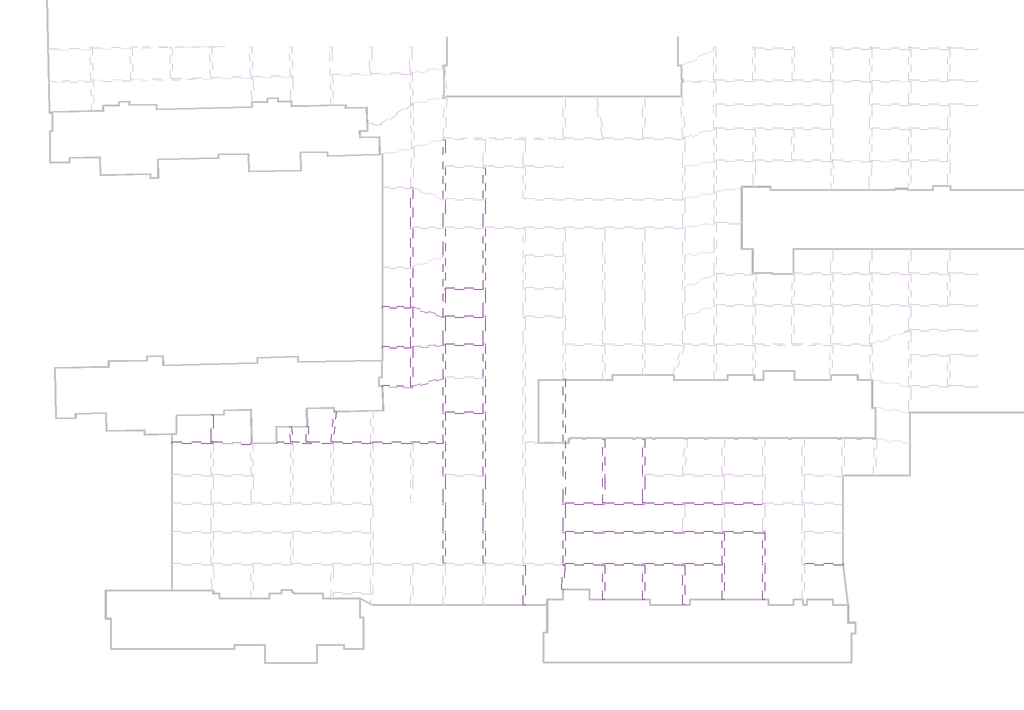
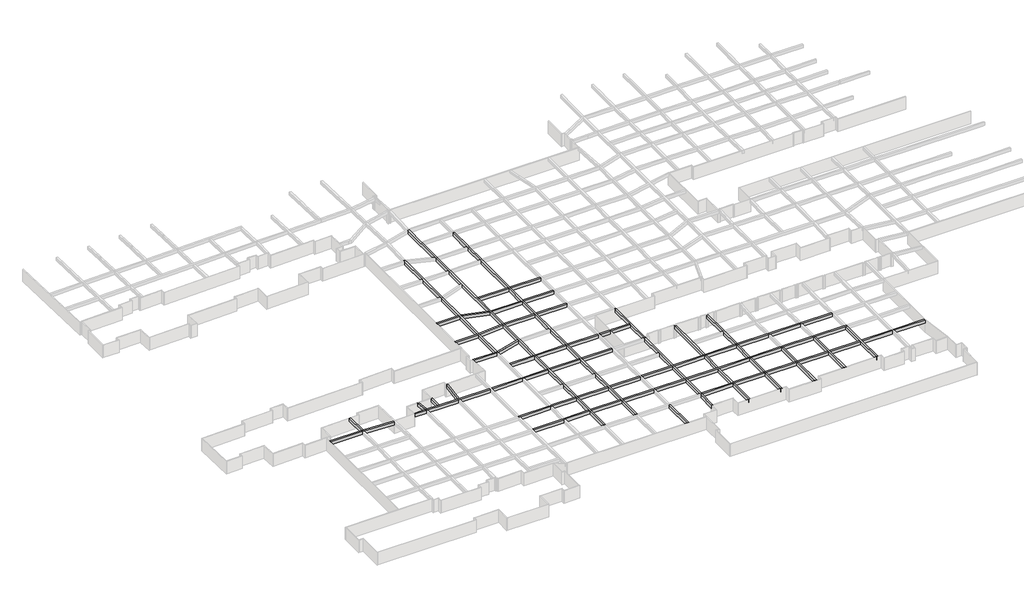
# One storey, part 9 of 20: 35 beams.
"""IFC4 building model written with IfcOpenShell, lengths in millimetres."""

from ifc_helpers import new_model, si_unit, frame, origin, place, context, project, spatial, polyline, outline, extrude, faceted_brep, element, save

model = new_model("IFC4")

# Units and contexts
model_context = context("Model", 3, world=origin())
ifc_project = project(units=[si_unit("LENGTHUNIT", "METRE", prefix="MILLI")], contexts=[model_context])

# Site, building, storey
site = spatial("IfcSite", under=ifc_project)
building = spatial("IfcBuilding", under=site)
storey = spatial("IfcBuildingStorey", under=building, Name="户型图", Elevation=0.0)

# Beams
placement = place(None, origin())
element("IfcBeam", 1, ObjectType="混凝土 - 矩形梁 : KL_beam", at=placement, inside=storey, context=model_context, shape_type="Brep", body=[
    faceted_brep([(62850.0, 87660.0, 3300.0), (62450.0, 87660.0, 3300.0), (62450.0, 81510.0, 3300.0), (62450.0, 81110.0, 3300.0), (62450.0, 75860.0, 3300.0), (62450.0, 75460.0, 3300.0), (62450.0, 63660.0, 3300.0), (62450.0, 63260.0, 3300.0), (62450.0, 57960.0, 3300.0), (62450.0, 57560.0, 3300.0), (62450.0, 52365.0, 3300.0), (62450.0, 51965.0, 3300.0), (62450.0, 45760.0, 3300.0), (62450.0, 45360.0, 3300.0), (62450.0, 38790.0, 3300.0), (62450.0, 38390.0, 3300.0), (62450.0, 32740.0, 3300.0), (62450.0, 32340.0, 3300.0), (62450.0, 26240.0, 3300.0), (62450.0, 25840.0, 3300.0), (62450.0, 20540.0, 3300.0), (62450.0, 20140.0, 3300.0), (62450.0, 14840.0, 3300.0), (62450.0, 14440.0, 3300.0), (62450.0, 8340.0, 3300.0), (62850.0, 8340.0, 3300.0), (62850.0, 14440.0, 3300.0), (62850.0, 14840.0, 3300.0), (62850.0, 20140.0, 3300.0), (62850.0, 20540.0, 3300.0), (62850.0, 25840.0, 3300.0), (62850.0, 26240.0, 3300.0), (62850.0, 32340.0, 3300.0), (62850.0, 32740.0, 3300.0), (62850.0, 38390.0, 3300.0), (62850.0, 38790.0, 3300.0), (62850.0, 45360.0, 3300.0), (62850.0, 45760.0, 3300.0), (62850.0, 51965.0, 3300.0), (62850.0, 52365.0, 3300.0), (62850.0, 57560.0, 3300.0), (62850.0, 57960.0, 3300.0), (62850.0, 63260.0, 3300.0), (62850.0, 63660.0, 3300.0), (62850.0, 75460.0, 3300.0), (62850.0, 75860.0, 3300.0), (62850.0, 81110.0, 3300.0), (62850.0, 81510.0, 3300.0), (62450.0, 87660.0, 2500.0), (62450.0, 81510.0, 2500.0), (62450.0, 81110.0, 2500.0), (62450.0, 75860.0, 2500.0), (62450.0, 75460.0, 2500.0), (62450.0, 63660.0, 2500.0), (62450.0, 63260.0, 2500.0), (62450.0, 57960.0, 2500.0), (62450.0, 57560.0, 2500.0), (62450.0, 52365.0, 2500.0), (62450.0, 51965.0, 2500.0), (62450.0, 45760.0, 2500.0), (62450.0, 45360.0, 2500.0), (62450.0, 38790.0, 2500.0), (62450.0, 38390.0, 2500.0), (62450.0, 32740.0, 2500.0), (62450.0, 32340.0, 2500.0), (62450.0, 26240.0, 2500.0), (62450.0, 25840.0, 2500.0), (62450.0, 20540.0, 2500.0), (62450.0, 20140.0, 2500.0), (62450.0, 14840.0, 2500.0), (62450.0, 14440.0, 2500.0), (62450.0, 8340.0, 2500.0), (62850.0, 87660.0, 2500.0), (62850.0, 81510.0, 2500.0), (62850.0, 81110.0, 2500.0), (62850.0, 75860.0, 2500.0), (62850.0, 75460.0, 2500.0), (62850.0, 63660.0, 2500.0), (62850.0, 63260.0, 2500.0), (62850.0, 57960.0, 2500.0), (62850.0, 57560.0, 2500.0), (62850.0, 52365.0, 2500.0), (62850.0, 51965.0, 2500.0), (62850.0, 45760.0, 2500.0), (62850.0, 45360.0, 2500.0), (62850.0, 38790.0, 2500.0), (62850.0, 38390.0, 2500.0), (62850.0, 32740.0, 2500.0), (62850.0, 32340.0, 2500.0), (62850.0, 26240.0, 2500.0), (62850.0, 25840.0, 2500.0), (62850.0, 20540.0, 2500.0), (62850.0, 20140.0, 2500.0), (62850.0, 14840.0, 2500.0), (62850.0, 14440.0, 2500.0), (62850.0, 8340.0, 2500.0)], [[[0, 1, 2, 3, 4, 5, 6, 7, 8, 9, 10, 11, 12, 13, 14, 15, 16, 17, 18, 19, 20, 21, 22, 23, 24, 25, 26, 27, 28, 29, 30, 31, 32, 33, 34, 35, 36, 37, 38, 39, 40, 41, 42, 43, 44, 45, 46, 47]], [[1, 48, 49, 50, 51, 52, 53, 54, 55, 56, 57, 58, 59, 60, 61, 62, 63, 64, 65, 66, 67, 68, 69, 70, 71, 24, 23, 22, 21, 20, 19, 18, 17, 16, 15, 14, 13, 12, 11, 10, 9, 8, 7, 6, 5, 4, 3, 2]], [[48, 72, 73, 74, 75, 76, 77, 78, 79, 80, 81, 82, 83, 84, 85, 86, 87, 88, 89, 90, 91, 92, 93, 94, 95, 71, 70, 69, 68, 67, 66, 65, 64, 63, 62, 61, 60, 59, 58, 57, 56, 55, 54, 53, 52, 51, 50, 49]], [[72, 0, 47, 46, 45, 44, 43, 42, 41, 40, 39, 38, 37, 36, 35, 34, 33, 32, 31, 30, 29, 28, 27, 26, 25, 95, 94, 93, 92, 91, 90, 89, 88, 87, 86, 85, 84, 83, 82, 81, 80, 79, 78, 77, 76, 75, 74, 73]], [[1, 0, 72, 48]], [[25, 24, 71, 95]]]),
])
element("IfcBeam", 2, ObjectType="混凝土 - 矩形梁 : KL_beam", at=placement, inside=storey, context=model_context, shape_type="Brep", body=[
    faceted_brep([(54850.0, 93310.0, 3300.0), (54450.0, 93310.0, 3300.0), (54450.0, 93242.5852338, 3300.0), (54450.0, 81594.9773948, 3300.0), (54450.0, 81169.6379898, 3300.0), (54450.0, 75860.0, 3300.0), (54450.0, 75460.0, 3300.0), (54450.0, 70165.8480304, 3300.0), (54450.0, 69740.1769214, 3300.0), (54450.0, 58026.8308056, 3300.0), (54450.0, 57610.0922713, 3300.0), (54450.0, 52350.0642398, 3300.0), (54450.0, 51948.8588371, 3300.0), (54450.0, 45709.9077287, 3300.0), (54450.0, 45293.1691944, 3300.0), (54450.0, 38790.0, 3300.0), (54450.0, 38390.0, 3300.0), (54450.0, 32740.0, 3300.0), (54450.0, 32340.0, 3300.0), (54450.0, 26240.0, 3300.0), (54450.0, 25840.0, 3300.0), (54450.0, 20540.0, 3300.0), (54450.0, 20140.0, 3300.0), (54450.0, 14840.0, 3300.0), (54450.0, 14440.0, 3300.0), (54450.0, 8340.0, 3300.0), (54850.0, 8340.0, 3300.0), (54850.0, 14440.0, 3300.0), (54850.0, 14840.0, 3300.0), (54850.0, 20140.0, 3300.0), (54850.0, 20540.0, 3300.0), (54850.0, 25840.0, 3300.0), (54850.0, 26240.0, 3300.0), (54850.0, 32340.0, 3300.0), (54850.0, 32740.0, 3300.0), (54850.0, 38390.0, 3300.0), (54850.0, 38790.0, 3300.0), (54850.0, 45360.0, 3300.0), (54850.0, 45760.0, 3300.0), (54850.0, 51965.0, 3300.0), (54850.0, 52365.0, 3300.0), (54850.0, 57560.0, 3300.0), (54850.0, 57960.0, 3300.0), (54850.0, 63260.0, 3300.0), (54850.0, 63660.0, 3300.0), (54850.0, 75460.0, 3300.0), (54850.0, 75860.0, 3300.0), (54850.0, 81110.0, 3300.0), (54850.0, 81510.0, 3300.0), (54850.0, 87660.0, 3300.0), (54850.0, 88060.0, 3300.0), (54850.0, 93310.0, 2500.0), (54850.0, 8340.0, 2500.0), (54850.0, 14440.0, 2500.0), (54850.0, 14840.0, 2500.0), (54850.0, 20140.0, 2500.0), (54850.0, 20540.0, 2500.0), (54850.0, 25840.0, 2500.0), (54850.0, 26240.0, 2500.0), (54850.0, 32340.0, 2500.0), (54850.0, 32740.0, 2500.0), (54850.0, 38390.0, 2500.0), (54850.0, 38790.0, 2500.0), (54850.0, 45360.0, 2500.0), (54850.0, 45760.0, 2500.0), (54850.0, 51965.0, 2500.0), (54850.0, 52365.0, 2500.0), (54850.0, 57560.0, 2500.0), (54850.0, 57960.0, 2500.0), (54850.0, 63260.0, 2500.0), (54850.0, 63660.0, 2500.0), (54850.0, 75460.0, 2500.0), (54850.0, 75860.0, 2500.0), (54850.0, 81110.0, 2500.0), (54850.0, 81510.0, 2500.0), (54850.0, 87660.0, 2500.0), (54850.0, 88060.0, 2500.0), (54450.0, 93310.0, 2500.0), (54450.0, 8340.0, 2500.0), (54450.0, 14440.0, 2500.0), (54450.0, 14840.0, 2500.0), (54450.0, 20140.0, 2500.0), (54450.0, 20540.0, 2500.0), (54450.0, 25840.0, 2500.0), (54450.0, 26240.0, 2500.0), (54450.0, 32340.0, 2500.0), (54450.0, 32740.0, 2500.0), (54450.0, 38390.0, 2500.0), (54450.0, 38790.0, 2500.0), (54450.0, 45293.1691944, 2500.0), (54450.0, 45709.9077287, 2500.0), (54450.0, 51948.8588371, 2500.0), (54450.0, 52350.0642398, 2500.0), (54450.0, 57610.0922713, 2500.0), (54450.0, 58026.8308056, 2500.0), (54450.0, 69740.1769214, 2500.0), (54450.0, 70165.8480304, 2500.0), (54450.0, 75460.0, 2500.0), (54450.0, 75860.0, 2500.0), (54450.0, 81169.6379898, 2500.0), (54450.0, 81594.9773948, 2500.0), (54450.0, 93242.5852338, 2500.0)], [[[0, 1, 2, 3, 4, 5, 6, 7, 8, 9, 10, 11, 12, 13, 14, 15, 16, 17, 18, 19, 20, 21, 22, 23, 24, 25, 26, 27, 28, 29, 30, 31, 32, 33, 34, 35, 36, 37, 38, 39, 40, 41, 42, 43, 44, 45, 46, 47, 48, 49, 50]], [[51, 0, 50, 49, 48, 47, 46, 45, 44, 43, 42, 41, 40, 39, 38, 37, 36, 35, 34, 33, 32, 31, 30, 29, 28, 27, 26, 52, 53, 54, 55, 56, 57, 58, 59, 60, 61, 62, 63, 64, 65, 66, 67, 68, 69, 70, 71, 72, 73, 74, 75, 76]], [[77, 51, 76, 75, 74, 73, 72, 71, 70, 69, 68, 67, 66, 65, 64, 63, 62, 61, 60, 59, 58, 57, 56, 55, 54, 53, 52, 78, 79, 80, 81, 82, 83, 84, 85, 86, 87, 88, 89, 90, 91, 92, 93, 94, 95, 96, 97, 98, 99, 100, 101]], [[1, 77, 101, 100, 99, 98, 97, 96, 95, 94, 93, 92, 91, 90, 89, 88, 87, 86, 85, 84, 83, 82, 81, 80, 79, 78, 25, 24, 23, 22, 21, 20, 19, 18, 17, 16, 15, 14, 13, 12, 11, 10, 9, 8, 7, 6, 5, 4, 3, 2]], [[1, 0, 51, 77]], [[26, 25, 78, 52]]]),
])
element("IfcBeam", 3, ObjectType="混凝土 - 矩形梁 : KL_beam", at=placement, inside=storey, context=model_context, shape_type="SweptSolid", body=[
    extrude(outline(polyline([(54850.0, 63260.0), (54850.0, 63660.0), (62450.0, 63660.0), (62450.0, 63260.0), (54850.0, 63260.0)])), frame((0.0, 0.0, 2500.0), z_axis=(0.0, 0.0, 1.0), x_axis=(1.0, 0.0, 0.0)), (0.0, 0.0, 1.0), 800.0),
    extrude(outline(polyline([(70450.0, 63660.0), (70450.0, 63260.0), (62850.0, 63260.0), (62850.0, 63660.0), (70450.0, 63660.0)])), frame((0.0, 0.0, 2500.0), z_axis=(0.0, 0.0, 1.0), x_axis=(1.0, 0.0, 0.0)), (0.0, 0.0, 1.0), 800.0),
])
element("IfcBeam", 4, ObjectType="混凝土 - 矩形梁 : KL_beam", at=placement, inside=storey, context=model_context, shape_type="SweptSolid", body=[
    extrude(outline(polyline([(70450.0, 57960.0), (70450.0, 57560.0), (62850.0, 57560.0), (62850.0, 57960.0), (70450.0, 57960.0)])), frame((0.0, 0.0, 2500.0), z_axis=(0.0, 0.0, 1.0), x_axis=(1.0, 0.0, 0.0)), (0.0, 0.0, 1.0), 800.0),
    extrude(outline(polyline([(54850.0, 57560.0), (54850.0, 57960.0), (62450.0, 57960.0), (62450.0, 57560.0), (54850.0, 57560.0)])), frame((0.0, 0.0, 2500.0), z_axis=(0.0, 0.0, 1.0), x_axis=(1.0, 0.0, 0.0)), (0.0, 0.0, 1.0), 800.0),
])
element("IfcBeam", 5, ObjectType="混凝土 - 矩形梁 : KL_beam", at=placement, inside=storey, context=model_context, shape_type="SweptSolid", body=[
    extrude(outline(polyline([(70450.0, 52365.0), (70450.0, 51965.0), (62850.0, 51965.0), (62850.0, 52365.0), (70450.0, 52365.0)])), frame((0.0, 0.0, 2500.0), z_axis=(0.0, 0.0, 1.0), x_axis=(1.0, 0.0, 0.0)), (0.0, 0.0, 1.0), 800.0),
    extrude(outline(polyline([(54850.0, 51965.0), (54850.0, 52365.0), (62450.0, 52365.0), (62450.0, 51965.0), (54850.0, 51965.0)])), frame((0.0, 0.0, 2500.0), z_axis=(0.0, 0.0, 1.0), x_axis=(1.0, 0.0, 0.0)), (0.0, 0.0, 1.0), 800.0),
])
element("IfcBeam", 6, ObjectType="混凝土 - 矩形梁 : KL_beam", at=placement, inside=storey, context=model_context, shape_type="Brep", body=[
    faceted_brep([(78450.0, 7940.0, 3300.0), (78841.1483464, 7940.0, 3300.0), (78850.0, 7940.0, 3300.0), (78850.0, 8340.0, 3300.0), (78850.0, 14440.0, 3300.0), (78850.0, 14840.0, 3300.0), (78850.0, 20140.0, 3300.0), (78850.0, 20540.0, 3300.0), (78850.0, 45360.0, 3300.0), (78450.0, 45360.0, 3300.0), (78450.0, 38790.0, 3300.0), (78450.0, 38390.0, 3300.0), (78450.0, 32740.0, 3300.0), (78450.0, 32340.0, 3300.0), (78450.0, 26240.0, 3300.0), (78450.0, 25840.0, 3300.0), (78450.0, 20540.0, 3300.0), (78450.0, 20140.0, 3300.0), (78450.0, 14840.0, 3300.0), (78450.0, 14440.0, 3300.0), (78450.0, 8340.0, 3300.0), (78450.0, 7940.0, 2500.0), (78450.0, 45360.0, 2500.0), (78450.0, 38790.0, 2500.0), (78450.0, 38390.0, 2500.0), (78450.0, 32740.0, 2500.0), (78450.0, 32340.0, 2500.0), (78450.0, 26240.0, 2500.0), (78450.0, 25840.0, 2500.0), (78450.0, 20540.0, 2500.0), (78450.0, 20140.0, 2500.0), (78450.0, 14840.0, 2500.0), (78450.0, 14440.0, 2500.0), (78450.0, 8340.0, 2500.0), (78850.0, 7940.0, 2500.0), (78841.1483464, 7940.0, 2500.0), (78850.0, 45360.0, 2500.0), (78850.0, 20540.0, 2500.0), (78850.0, 20140.0, 2500.0), (78850.0, 14840.0, 2500.0), (78850.0, 14440.0, 2500.0), (78850.0, 8340.0, 2500.0)], [[[0, 1, 2, 3, 4, 5, 6, 7, 8, 9, 10, 11, 12, 13, 14, 15, 16, 17, 18, 19, 20]], [[21, 0, 20, 19, 18, 17, 16, 15, 14, 13, 12, 11, 10, 9, 22, 23, 24, 25, 26, 27, 28, 29, 30, 31, 32, 33]], [[34, 35, 21, 33, 32, 31, 30, 29, 28, 27, 26, 25, 24, 23, 22, 36, 37, 38, 39, 40, 41]], [[2, 34, 41, 40, 39, 38, 37, 36, 8, 7, 6, 5, 4, 3]], [[9, 8, 36, 22]], [[2, 1, 0, 21, 35, 34]]]),
])
element("IfcBeam", 7, ObjectType="混凝土 - 矩形梁 : KL_beam", at=placement, inside=storey, context=model_context, shape_type="Brep", body=[
    faceted_brep([(54450.0, 14440.0, 3300.0), (54450.0, 14840.0, 3300.0), (48350.0, 14840.0, 3300.0), (47950.0, 14840.0, 3300.0), (40351.7306283, 14840.0, 3300.0), (40351.7306283, 14440.0, 3300.0), (47950.0, 14440.0, 3300.0), (48350.0, 14440.0, 3300.0), (54450.0, 14440.0, 2500.0), (40351.7306283, 14440.0, 2500.0), (47950.0, 14440.0, 2500.0), (48350.0, 14440.0, 2500.0), (54450.0, 14840.0, 2500.0), (40351.7306283, 14840.0, 2500.0), (47950.0, 14840.0, 2500.0), (48350.0, 14840.0, 2500.0)], [[[0, 1, 2, 3, 4, 5, 6, 7]], [[8, 0, 7, 6, 5, 9, 10, 11]], [[12, 8, 11, 10, 9, 13, 14, 15]], [[1, 12, 15, 14, 13, 4, 3, 2]], [[1, 0, 8, 12]], [[5, 4, 13, 9]]]),
    faceted_brep([(70450.0, 14840.0, 3300.0), (70450.0, 14440.0, 3300.0), (70450.0, 14440.0, 2500.0), (70450.0, 14840.0, 2500.0), (62850.0, 14440.0, 3300.0), (62850.0, 14840.0, 3300.0), (62850.0, 14840.0, 2500.0), (62850.0, 14440.0, 2500.0)], [[[0, 1, 2, 3]], [[4, 5, 6, 7]], [[1, 0, 5, 4]], [[2, 1, 4, 7]], [[3, 2, 7, 6]], [[0, 3, 6, 5]]]),
    faceted_brep([(70850.0, 14440.0, 3300.0), (70850.0, 14840.0, 3300.0), (70850.0, 14840.0, 2500.0), (70850.0, 14440.0, 2500.0), (78450.0, 14840.0, 3300.0), (78450.0, 14440.0, 3300.0), (78450.0, 14440.0, 2500.0), (78450.0, 14840.0, 2500.0)], [[[0, 1, 2, 3]], [[4, 5, 6, 7]], [[1, 0, 5, 4]], [[0, 3, 6, 5]], [[3, 2, 7, 6]], [[2, 1, 4, 7]]]),
    faceted_brep([(118850.0, 14440.0, 3300.0), (118850.0, 14840.0, 3300.0), (118450.0, 14840.0, 3300.0), (110824.4938701, 14840.0, 3300.0), (110424.4938701, 14840.0, 3300.0), (102834.0, 14840.0, 3300.0), (102434.0, 14840.0, 3300.0), (94845.0, 14840.0, 3300.0), (94445.0, 14840.0, 3300.0), (86850.0, 14840.0, 3300.0), (86450.0, 14840.0, 3300.0), (78850.0, 14840.0, 3300.0), (78850.0, 14440.0, 3300.0), (86450.0, 14440.0, 3300.0), (86850.0, 14440.0, 3300.0), (94445.0, 14440.0, 3300.0), (94845.0, 14440.0, 3300.0), (102434.0, 14440.0, 3300.0), (102834.0, 14440.0, 3300.0), (110424.4938701, 14440.0, 3300.0), (110824.4938701, 14440.0, 3300.0), (118450.0, 14440.0, 3300.0), (118850.0, 14440.0, 2500.0), (78850.0, 14440.0, 2500.0), (86450.0, 14440.0, 2500.0), (86850.0, 14440.0, 2500.0), (94445.0, 14440.0, 2500.0), (94845.0, 14440.0, 2500.0), (102434.0, 14440.0, 2500.0), (102834.0, 14440.0, 2500.0), (110424.4938701, 14440.0, 2500.0), (110824.4938701, 14440.0, 2500.0), (118450.0, 14440.0, 2500.0), (118850.0, 14840.0, 2500.0), (78850.0, 14840.0, 2500.0), (86450.0, 14840.0, 2500.0), (86850.0, 14840.0, 2500.0), (94445.0, 14840.0, 2500.0), (94845.0, 14840.0, 2500.0), (102434.0, 14840.0, 2500.0), (102834.0, 14840.0, 2500.0), (110424.4938701, 14840.0, 2500.0), (110824.4938701, 14840.0, 2500.0), (118450.0, 14840.0, 2500.0)], [[[0, 1, 2, 3, 4, 5, 6, 7, 8, 9, 10, 11, 12, 13, 14, 15, 16, 17, 18, 19, 20, 21]], [[22, 0, 21, 20, 19, 18, 17, 16, 15, 14, 13, 12, 23, 24, 25, 26, 27, 28, 29, 30, 31, 32]], [[33, 22, 32, 31, 30, 29, 28, 27, 26, 25, 24, 23, 34, 35, 36, 37, 38, 39, 40, 41, 42, 43]], [[1, 33, 43, 42, 41, 40, 39, 38, 37, 36, 35, 34, 11, 10, 9, 8, 7, 6, 5, 4, 3, 2]], [[12, 11, 34, 23]], [[1, 0, 22, 33]]]),
    faceted_brep([(62450.0, 14840.0, 3300.0), (62450.0, 14440.0, 3300.0), (62450.0, 14440.0, 2500.0), (62450.0, 14840.0, 2500.0), (54850.0, 14440.0, 3300.0), (54850.0, 14840.0, 3300.0), (54850.0, 14840.0, 2500.0), (54850.0, 14440.0, 2500.0)], [[[0, 1, 2, 3]], [[4, 5, 6, 7]], [[1, 0, 5, 4]], [[2, 1, 4, 7]], [[3, 2, 7, 6]], [[0, 3, 6, 5]]]),
])
element("IfcBeam", 8, ObjectType="混凝土 - 矩形梁 : KL_beam", at=placement, inside=storey, context=model_context, shape_type="Brep", body=[
    faceted_brep([(39951.7306283, 20540.0, 3300.0), (39951.7306283, 20140.0, 3300.0), (40351.7306283, 20140.0, 3300.0), (47950.0, 20140.0, 3300.0), (48350.0, 20140.0, 3300.0), (54450.0, 20140.0, 3300.0), (54450.0, 20540.0, 3300.0), (48350.0, 20540.0, 3300.0), (47950.0, 20540.0, 3300.0), (40351.7306283, 20540.0, 3300.0), (39951.7306283, 20140.0, 2500.0), (40351.7306283, 20140.0, 2500.0), (47950.0, 20140.0, 2500.0), (48350.0, 20140.0, 2500.0), (54450.0, 20140.0, 2500.0), (39951.7306283, 20540.0, 2500.0), (40351.7306283, 20540.0, 2500.0), (47950.0, 20540.0, 2500.0), (48350.0, 20540.0, 2500.0), (54450.0, 20540.0, 2500.0)], [[[0, 1, 2, 3, 4, 5, 6, 7, 8, 9]], [[1, 10, 11, 12, 13, 14, 5, 4, 3, 2]], [[10, 15, 16, 17, 18, 19, 14, 13, 12, 11]], [[15, 0, 9, 8, 7, 6, 19, 18, 17, 16]], [[6, 5, 14, 19]], [[1, 0, 15, 10]]]),
    faceted_brep([(70450.0, 20540.0, 3300.0), (70450.0, 20140.0, 3300.0), (70450.0, 20140.0, 2500.0), (70450.0, 20540.0, 2500.0), (62850.0, 20140.0, 3300.0), (62850.0, 20540.0, 3300.0), (62850.0, 20540.0, 2500.0), (62850.0, 20140.0, 2500.0)], [[[0, 1, 2, 3]], [[4, 5, 6, 7]], [[1, 0, 5, 4]], [[2, 1, 4, 7]], [[3, 2, 7, 6]], [[0, 3, 6, 5]]]),
    faceted_brep([(70850.0, 20140.0, 3300.0), (70850.0, 20540.0, 3300.0), (70850.0, 20540.0, 2500.0), (70850.0, 20140.0, 2500.0), (78450.0, 20540.0, 3300.0), (78450.0, 20140.0, 3300.0), (78450.0, 20140.0, 2500.0), (78450.0, 20540.0, 2500.0)], [[[0, 1, 2, 3]], [[4, 5, 6, 7]], [[1, 0, 5, 4]], [[0, 3, 6, 5]], [[3, 2, 7, 6]], [[2, 1, 4, 7]]]),
    faceted_brep([(78850.0, 20540.0, 3300.0), (78850.0, 20140.0, 3300.0), (86450.0, 20140.0, 3300.0), (86850.0, 20140.0, 3300.0), (94445.0, 20140.0, 3300.0), (94845.0, 20140.0, 3300.0), (102434.0, 20140.0, 3300.0), (102834.0, 20140.0, 3300.0), (110424.4938701, 20140.0, 3300.0), (110824.4938701, 20140.0, 3300.0), (118450.0, 20140.0, 3300.0), (118450.0, 20540.0, 3300.0), (110821.0333227, 20540.0, 3300.0), (110420.9723915, 20540.0, 3300.0), (102834.0, 20540.0, 3300.0), (102434.0, 20540.0, 3300.0), (94845.0, 20540.0, 3300.0), (94445.0, 20540.0, 3300.0), (86850.0, 20540.0, 3300.0), (86450.0, 20540.0, 3300.0), (78850.0, 20140.0, 2500.0), (86450.0, 20140.0, 2500.0), (86850.0, 20140.0, 2500.0), (94445.0, 20140.0, 2500.0), (94845.0, 20140.0, 2500.0), (102434.0, 20140.0, 2500.0), (102834.0, 20140.0, 2500.0), (110424.4938701, 20140.0, 2500.0), (110824.4938701, 20140.0, 2500.0), (118450.0, 20140.0, 2500.0), (78850.0, 20540.0, 2500.0), (86450.0, 20540.0, 2500.0), (86850.0, 20540.0, 2500.0), (94445.0, 20540.0, 2500.0), (94845.0, 20540.0, 2500.0), (102434.0, 20540.0, 2500.0), (102834.0, 20540.0, 2500.0), (110420.9723915, 20540.0, 2500.0), (110821.0333227, 20540.0, 2500.0), (118450.0, 20540.0, 2500.0)], [[[0, 1, 2, 3, 4, 5, 6, 7, 8, 9, 10, 11, 12, 13, 14, 15, 16, 17, 18, 19]], [[1, 20, 21, 22, 23, 24, 25, 26, 27, 28, 29, 10, 9, 8, 7, 6, 5, 4, 3, 2]], [[20, 30, 31, 32, 33, 34, 35, 36, 37, 38, 39, 29, 28, 27, 26, 25, 24, 23, 22, 21]], [[30, 0, 19, 18, 17, 16, 15, 14, 13, 12, 11, 39, 38, 37, 36, 35, 34, 33, 32, 31]], [[1, 0, 30, 20]], [[11, 10, 29, 39]]]),
    faceted_brep([(62450.0, 20540.0, 3300.0), (62450.0, 20140.0, 3300.0), (62450.0, 20140.0, 2500.0), (62450.0, 20540.0, 2500.0), (54850.0, 20140.0, 3300.0), (54850.0, 20540.0, 3300.0), (54850.0, 20540.0, 2500.0), (54850.0, 20140.0, 2500.0)], [[[0, 1, 2, 3]], [[4, 5, 6, 7]], [[1, 0, 5, 4]], [[2, 1, 4, 7]], [[3, 2, 7, 6]], [[0, 3, 6, 5]]]),
])
element("IfcBeam", 9, ObjectType="混凝土 - 矩形梁 : KL_beam", at=placement, inside=storey, context=model_context, shape_type="Brep", body=[
    faceted_brep([(54450.0, 32340.0, 3300.0), (54450.0, 32740.0, 3300.0), (48350.0, 32740.0, 3300.0), (47950.0, 32740.0, 3300.0), (40351.7306283, 32740.0, 3300.0), (40351.7306283, 32340.0, 3300.0), (47950.0, 32340.0, 3300.0), (48350.0, 32340.0, 3300.0), (54450.0, 32340.0, 2500.0), (40351.7306283, 32340.0, 2500.0), (47950.0, 32340.0, 2500.0), (48350.0, 32340.0, 2500.0), (54450.0, 32740.0, 2500.0), (40351.7306283, 32740.0, 2500.0), (47950.0, 32740.0, 2500.0), (48350.0, 32740.0, 2500.0)], [[[0, 1, 2, 3, 4, 5, 6, 7]], [[8, 0, 7, 6, 5, 9, 10, 11]], [[12, 8, 11, 10, 9, 13, 14, 15]], [[1, 12, 15, 14, 13, 4, 3, 2]], [[1, 0, 8, 12]], [[5, 4, 13, 9]]]),
    faceted_brep([(70450.0, 32740.0, 3300.0), (70450.0, 32340.0, 3300.0), (70450.0, 32340.0, 2500.0), (70450.0, 32740.0, 2500.0), (62850.0, 32340.0, 3300.0), (62850.0, 32740.0, 3300.0), (62850.0, 32740.0, 2500.0), (62850.0, 32340.0, 2500.0)], [[[0, 1, 2, 3]], [[4, 5, 6, 7]], [[1, 0, 5, 4]], [[2, 1, 4, 7]], [[3, 2, 7, 6]], [[0, 3, 6, 5]]]),
    faceted_brep([(62450.0, 32740.0, 3300.0), (62450.0, 32340.0, 3300.0), (62450.0, 32340.0, 2500.0), (62450.0, 32740.0, 2500.0), (54850.0, 32340.0, 3300.0), (54850.0, 32740.0, 3300.0), (54850.0, 32740.0, 2500.0), (54850.0, 32340.0, 2500.0)], [[[0, 1, 2, 3]], [[4, 5, 6, 7]], [[1, 0, 5, 4]], [[2, 1, 4, 7]], [[3, 2, 7, 6]], [[0, 3, 6, 5]]]),
])
element("IfcBeam", 10, ObjectType="混凝土 - 矩形梁 : KL_beam", at=placement, inside=storey, context=model_context, shape_type="SweptSolid", body=[
    extrude(outline(polyline([(54450.0, 38790.0), (54450.0, 38390.0), (48350.0, 38390.0), (48350.0, 38790.0), (54450.0, 38790.0)])), frame((0.0, 0.0, 2500.0), z_axis=(0.0, 0.0, 1.0), x_axis=(1.0, 0.0, 0.0)), (0.0, 0.0, 1.0), 800.0),
    extrude(outline(polyline([(78450.0, 38790.0), (78450.0, 38390.0), (70850.0, 38390.0), (70850.0, 38790.0), (78450.0, 38790.0)])), frame((0.0, 0.0, 2500.0), z_axis=(0.0, 0.0, 1.0), x_axis=(1.0, 0.0, 0.0)), (0.0, 0.0, 1.0), 800.0),
    extrude(outline(polyline([(70450.0, 38790.0), (70450.0, 38390.0), (62850.0, 38390.0), (62850.0, 38790.0), (70450.0, 38790.0)])), frame((0.0, 0.0, 2500.0), z_axis=(0.0, 0.0, 1.0), x_axis=(1.0, 0.0, 0.0)), (0.0, 0.0, 1.0), 800.0),
    extrude(outline(polyline([(62450.0, 38790.0), (62450.0, 38390.0), (54850.0, 38390.0), (54850.0, 38790.0), (62450.0, 38790.0)])), frame((0.0, 0.0, 2500.0), z_axis=(0.0, 0.0, 1.0), x_axis=(1.0, 0.0, 0.0)), (0.0, 0.0, 1.0), 800.0),
])
element("IfcBeam", 11, ObjectType="混凝土 - 矩形梁 : KL_beam", at=placement, inside=storey, context=model_context, shape_type="Brep", body=[
    faceted_brep([(86850.0, 33258.0, 3300.0), (86850.0, 33258.0, 2500.0), (86450.0, 33258.0, 2500.0), (86450.0, 33258.0, 3300.0), (86850.0, 20540.0, 3300.0), (86450.0, 20540.0, 3300.0), (86450.0, 20540.0, 2500.0), (86850.0, 20540.0, 2500.0), (86850.0, 25840.0, 3300.0), (86850.0, 26240.0, 3300.0), (86850.0, 26240.0, 2500.0), (86850.0, 25840.0, 2500.0)], [[[0, 1, 2, 3]], [[4, 5, 6, 7]], [[0, 3, 5, 4, 8, 9]], [[3, 2, 6, 5]], [[2, 1, 10, 11, 7, 6]], [[1, 0, 9, 8, 4, 7, 11, 10]]]),
    faceted_brep([(86450.0, 14840.0, 3300.0), (86850.0, 14840.0, 3300.0), (86850.0, 20140.0, 3300.0), (86450.0, 20140.0, 3300.0), (86450.0, 14840.0, 2500.0), (86450.0, 20140.0, 2500.0), (86850.0, 14840.0, 2500.0), (86850.0, 20140.0, 2500.0)], [[[0, 1, 2, 3]], [[4, 0, 3, 5]], [[6, 4, 5, 7]], [[1, 6, 7, 2]], [[1, 0, 4, 6]], [[3, 2, 7, 5]]]),
])
element("IfcBeam", 12, ObjectType="混凝土 - 矩形梁 : KL_beam", at=placement, inside=storey, context=model_context, shape_type="Brep", body=[
    faceted_brep([(94845.0, 33257.0, 3300.0), (94845.0, 33257.0, 2500.0), (94445.0, 33257.0, 2500.0), (94445.0, 33257.0, 3300.0), (94845.0, 20540.0, 3300.0), (94445.0, 20540.0, 3300.0), (94445.0, 20540.0, 2500.0), (94845.0, 20540.0, 2500.0), (94445.0, 26240.0, 3300.0), (94445.0, 25840.0, 3300.0), (94845.0, 25840.0, 3300.0), (94845.0, 26240.0, 3300.0), (94445.0, 26240.0, 2500.0), (94445.0, 25840.0, 2500.0), (94845.0, 26240.0, 2500.0), (94845.0, 25840.0, 2500.0)], [[[0, 1, 2, 3]], [[4, 5, 6, 7]], [[0, 3, 8, 9, 5, 4, 10, 11]], [[3, 2, 12, 13, 6, 5, 9, 8]], [[2, 1, 14, 15, 7, 6, 13, 12]], [[1, 0, 11, 10, 4, 7, 15, 14]]]),
    faceted_brep([(94445.0, 14840.0, 3300.0), (94845.0, 14840.0, 3300.0), (94845.0, 20140.0, 3300.0), (94445.0, 20140.0, 3300.0), (94445.0, 14840.0, 2500.0), (94445.0, 20140.0, 2500.0), (94845.0, 14840.0, 2500.0), (94845.0, 20140.0, 2500.0)], [[[0, 1, 2, 3]], [[4, 0, 3, 5]], [[6, 4, 5, 7]], [[1, 6, 7, 2]], [[1, 0, 4, 6]], [[3, 2, 7, 5]]]),
])
element("IfcBeam", 13, ObjectType="混凝土 - 矩形梁 : KL_beam", at=placement, inside=storey, context=model_context, shape_type="Brep", body=[
    faceted_brep([(118850.0, 1106.0, 3300.0), (118450.0, 1106.0, 3300.0), (118450.0, 1106.0, 2500.0), (118850.0, 1106.0, 2500.0), (118850.0, 7940.0, 3300.0), (118850.0, 8340.0, 3300.0), (118850.0, 14440.0, 3300.0), (118450.0, 14440.0, 3300.0), (118450.0, 8340.0, 3300.0), (118450.0, 7940.0, 3300.0), (118450.0, 14440.0, 2500.0), (118450.0, 8340.0, 2500.0), (118450.0, 7940.0, 2500.0), (118850.0, 14440.0, 2500.0), (118850.0, 8340.0, 2500.0), (118850.0, 7940.0, 2500.0)], [[[0, 1, 2, 3]], [[1, 0, 4, 5, 6, 7, 8, 9]], [[2, 1, 9, 8, 7, 10, 11, 12]], [[3, 2, 12, 11, 10, 13, 14, 15]], [[0, 3, 15, 14, 13, 6, 5, 4]], [[7, 6, 13, 10]]]),
])
element("IfcBeam", 14, ObjectType="混凝土 - 矩形梁 : KL_beam", at=placement, inside=storey, context=model_context, shape_type="SweptSolid", body=[
    extrude(outline(polyline([(134623.6143656, 8340.0), (134623.6143656, 7940.0), (126844.0, 7940.0), (126844.0, 8340.0), (134623.6143656, 8340.0)])), frame((0.0, 0.0, 2500.0), z_axis=(0.0, 0.0, 1.0), x_axis=(1.0, 0.0, 0.0)), (0.0, 0.0, 1.0), 800.0),
    extrude(outline(polyline([(126444.0, 8340.0), (126444.0, 7940.0), (118850.0, 7940.0), (118850.0, 8340.0), (126444.0, 8340.0)])), frame((0.0, 0.0, 2500.0), z_axis=(0.0, 0.0, 1.0), x_axis=(1.0, 0.0, 0.0)), (0.0, 0.0, 1.0), 800.0),
    extrude(outline(polyline([(118450.0, 8340.0), (118450.0, 7940.0), (110824.4938701, 7940.0), (110824.4938701, 8340.0), (118450.0, 8340.0)])), frame((0.0, 0.0, 2500.0), z_axis=(0.0, 0.0, 1.0), x_axis=(1.0, 0.0, 0.0)), (0.0, 0.0, 1.0), 800.0),
])
element("IfcBeam", 15, ObjectType="混凝土 - 矩形梁 : KL_beam", at=placement, inside=storey, context=model_context, shape_type="Brep", body=[
    faceted_brep([(110824.4938701, 1106.0, 3300.0), (110424.4938701, 1106.0, 3300.0), (110424.4938701, 1106.0, 2500.0), (110824.4938701, 1106.0, 2500.0), (110824.4938701, 7940.0, 3300.0), (110824.4938701, 8340.0, 3300.0), (110824.4938701, 14440.0, 3300.0), (110424.4938701, 14440.0, 3300.0), (110424.4938701, 8340.0, 3300.0), (110424.4938701, 7940.0, 3300.0), (110424.4938701, 14440.0, 2500.0), (110424.4938701, 8340.0, 2500.0), (110424.4938701, 7940.0, 2500.0), (110824.4938701, 14440.0, 2500.0), (110824.4938701, 8340.0, 2500.0), (110824.4938701, 7940.0, 2500.0)], [[[0, 1, 2, 3]], [[1, 0, 4, 5, 6, 7, 8, 9]], [[2, 1, 9, 8, 7, 10, 11, 12]], [[3, 2, 12, 11, 10, 13, 14, 15]], [[0, 3, 15, 14, 13, 6, 5, 4]], [[7, 6, 13, 10]]]),
])
element("IfcBeam", 16, ObjectType="混凝土 - 矩形梁 : KL_beam", at=placement, inside=storey, context=model_context, shape_type="Brep", body=[
    faceted_brep([(78850.0, 8340.0, 3300.0), (78850.0, 7940.0, 3300.0), (86450.0, 7940.0, 3300.0), (86850.0, 7940.0, 3300.0), (94445.0, 7940.0, 3300.0), (94845.0, 7940.0, 3300.0), (102434.0, 7940.0, 3300.0), (102834.0, 7940.0, 3300.0), (110424.4938701, 7940.0, 3300.0), (110424.4938701, 8340.0, 3300.0), (102834.0, 8340.0, 3300.0), (102434.0, 8340.0, 3300.0), (94845.0, 8340.0, 3300.0), (94445.0, 8340.0, 3300.0), (86850.0, 8340.0, 3300.0), (86450.0, 8340.0, 3300.0), (78850.0, 7940.0, 2500.0), (86450.0, 7940.0, 2500.0), (86850.0, 7940.0, 2500.0), (94445.0, 7940.0, 2500.0), (94845.0, 7940.0, 2500.0), (102434.0, 7940.0, 2500.0), (102834.0, 7940.0, 2500.0), (110424.4938701, 7940.0, 2500.0), (78850.0, 8340.0, 2500.0), (86450.0, 8340.0, 2500.0), (86850.0, 8340.0, 2500.0), (94445.0, 8340.0, 2500.0), (94845.0, 8340.0, 2500.0), (102434.0, 8340.0, 2500.0), (102834.0, 8340.0, 2500.0), (110424.4938701, 8340.0, 2500.0)], [[[0, 1, 2, 3, 4, 5, 6, 7, 8, 9, 10, 11, 12, 13, 14, 15]], [[1, 16, 17, 18, 19, 20, 21, 22, 23, 8, 7, 6, 5, 4, 3, 2]], [[16, 24, 25, 26, 27, 28, 29, 30, 31, 23, 22, 21, 20, 19, 18, 17]], [[24, 0, 15, 14, 13, 12, 11, 10, 9, 31, 30, 29, 28, 27, 26, 25]], [[1, 0, 24, 16]], [[9, 8, 23, 31]]]),
])
element("IfcBeam", 17, ObjectType="混凝土 - 矩形梁 : KL_beam", at=placement, inside=storey, context=model_context, shape_type="SweptSolid", body=[
    extrude(outline(polyline([(94845.0, 1106.0), (94445.0, 1106.0), (94445.0, 7940.0), (94845.0, 7940.0), (94845.0, 1106.0)])), frame((0.0, 0.0, 2500.0), z_axis=(0.0, 0.0, 1.0), x_axis=(1.0, 0.0, 0.0)), (0.0, 0.0, 1.0), 800.0),
    extrude(outline(polyline([(94445.0, 14440.0), (94845.0, 14440.0), (94845.0, 8340.0), (94445.0, 8340.0), (94445.0, 14440.0)])), frame((0.0, 0.0, 2500.0), z_axis=(0.0, 0.0, 1.0), x_axis=(1.0, 0.0, 0.0)), (0.0, 0.0, 1.0), 800.0),
])
element("IfcBeam", 18, ObjectType="混凝土 - 矩形梁 : KL_beam", at=placement, inside=storey, context=model_context, shape_type="SweptSolid", body=[
    extrude(outline(polyline([(102834.0, 40.0), (102434.0, 40.0), (102434.0, 7940.0), (102834.0, 7940.0), (102834.0, 40.0)])), frame((0.0, 0.0, 2500.0), z_axis=(0.0, 0.0, 1.0), x_axis=(1.0, 0.0, 0.0)), (0.0, 0.0, 1.0), 800.0),
    extrude(outline(polyline([(102434.0, 14440.0), (102834.0, 14440.0), (102834.0, 8340.0), (102434.0, 8340.0), (102434.0, 14440.0)])), frame((0.0, 0.0, 2500.0), z_axis=(0.0, 0.0, 1.0), x_axis=(1.0, 0.0, 0.0)), (0.0, 0.0, 1.0), 800.0),
])
element("IfcBeam", 19, ObjectType="混凝土 - 矩形梁 : KL_beam", at=placement, inside=storey, context=model_context, shape_type="SweptSolid", body=[
    extrude(outline(polyline([(86850.0, 1106.0), (86450.0, 1106.0), (86450.0, 7940.0), (86850.0, 7940.0), (86850.0, 1106.0)])), frame((0.0, 0.0, 2500.0), z_axis=(0.0, 0.0, 1.0), x_axis=(1.0, 0.0, 0.0)), (0.0, 0.0, 1.0), 800.0),
    extrude(outline(polyline([(86450.0, 14440.0), (86850.0, 14440.0), (86850.0, 8340.0), (86450.0, 8340.0), (86450.0, 14440.0)])), frame((0.0, 0.0, 2500.0), z_axis=(0.0, 0.0, 1.0), x_axis=(1.0, 0.0, 0.0)), (0.0, 0.0, 1.0), 800.0),
])
element("IfcBeam", 20, ObjectType="混凝土 - 矩形梁 : KL_beam", at=placement, inside=storey, context=model_context, shape_type="Brep", body=[
    faceted_brep([(21150.3653142, 32340.0, 3300.0), (21150.3653142, 32740.0, 3300.0), (21150.3653142, 32740.0, 2500.0), (21150.3653142, 32340.0, 2500.0), (23892.5739519, 32340.0, 3300.0), (24292.5739519, 32340.0, 3300.0), (31950.0, 32340.0, 3300.0), (32350.0, 32340.0, 3300.0), (39951.7306283, 32340.0, 3300.0), (39951.7306283, 32740.0, 3300.0), (32371.1565283, 32740.0, 3300.0), (31969.1326283, 32740.0, 3300.0), (27412.5739519, 32740.0, 3300.0), (27012.5739519, 32740.0, 3300.0), (24275.8401867, 32740.0, 3300.0), (23874.3122516, 32740.0, 3300.0), (39951.7306283, 32740.0, 2500.0), (32371.1565283, 32740.0, 2500.0), (31969.1326283, 32740.0, 2500.0), (27412.5739519, 32740.0, 2500.0), (27012.5739519, 32740.0, 2500.0), (24275.8401867, 32740.0, 2500.0), (23874.3122516, 32740.0, 2500.0), (39951.7306283, 32340.0, 2500.0), (32350.0, 32340.0, 2500.0), (31950.0, 32340.0, 2500.0), (24292.5739519, 32340.0, 2500.0), (23892.5739519, 32340.0, 2500.0)], [[[0, 1, 2, 3]], [[1, 0, 4, 5, 6, 7, 8, 9, 10, 11, 12, 13, 14, 15]], [[2, 1, 15, 14, 13, 12, 11, 10, 9, 16, 17, 18, 19, 20, 21, 22]], [[3, 2, 22, 21, 20, 19, 18, 17, 16, 23, 24, 25, 26, 27]], [[0, 3, 27, 26, 25, 24, 23, 8, 7, 6, 5, 4]], [[9, 8, 23, 16]]]),
])
element("IfcBeam", 21, ObjectType="混凝土 - 矩形梁 : KL_beam", at=placement, inside=storey, context=model_context, shape_type="SweptSolid", body=[
    extrude(outline(polyline([(32577.9819548, 38784.7959442), (32975.9682437, 38744.7096144), (32371.1565283, 32740.0), (31969.1326283, 32740.0), (32577.9819548, 38784.7959442)])), frame((0.0, 0.0, 2500.0), z_axis=(0.0, 0.0, 1.0), x_axis=(1.0, 0.0, 0.0)), (0.0, 0.0, 1.0), 800.0),
])
element("IfcBeam", 22, ObjectType="混凝土 - 矩形梁 : KL_beam", at=placement, inside=storey, context=model_context, shape_type="Brep", body=[
    faceted_brep([(48350.0, 83800.3620102, 3300.0), (47953.7843446, 83800.3620102, 3300.0), (47950.0, 83800.3620102, 3300.0), (47950.0, 83662.7494803, 3300.0), (47950.0, 83460.0, 3300.0), (47950.0, 75860.0, 3300.0), (47950.0, 75460.0, 3300.0), (47950.0, 67860.0, 3300.0), (47950.0, 67460.0, 3300.0), (47950.0, 59860.0, 3300.0), (47950.0, 59460.0, 3300.0), (47950.0, 51860.0, 3300.0), (47950.0, 51460.0, 3300.0), (47950.0, 43867.507495, 3300.0), (48350.0, 43852.7641216, 3300.0), (48350.0, 43926.8308056, 3300.0), (48350.0, 51474.9357602, 3300.0), (48350.0, 51876.1411629, 3300.0), (48350.0, 59393.1691944, 3300.0), (48350.0, 59809.9077287, 3300.0), (48350.0, 67519.9584924, 3300.0), (48350.0, 67945.6296013, 3300.0), (48350.0, 75460.0, 3300.0), (48350.0, 75860.0, 3300.0), (48350.0, 83375.0226052, 3300.0), (48350.0, 83800.3620102, 2500.0), (48350.0, 43852.7641216, 2500.0), (48350.0, 43926.8308056, 2500.0), (48350.0, 51474.9357602, 2500.0), (48350.0, 51876.1411629, 2500.0), (48350.0, 59393.1691944, 2500.0), (48350.0, 59809.9077287, 2500.0), (48350.0, 67519.9584924, 2500.0), (48350.0, 67945.6296013, 2500.0), (48350.0, 75460.0, 2500.0), (48350.0, 75860.0, 2500.0), (48350.0, 83375.0226052, 2500.0), (47950.0, 83800.3620102, 2500.0), (47953.7843446, 83800.3620102, 2500.0), (47950.0, 43867.507495, 2500.0), (47950.0, 51460.0, 2500.0), (47950.0, 51860.0, 2500.0), (47950.0, 59460.0, 2500.0), (47950.0, 59860.0, 2500.0), (47950.0, 67460.0, 2500.0), (47950.0, 67860.0, 2500.0), (47950.0, 75460.0, 2500.0), (47950.0, 75860.0, 2500.0), (47950.0, 83460.0, 2500.0), (47950.0, 83662.7494803, 2500.0)], [[[0, 1, 2, 3, 4, 5, 6, 7, 8, 9, 10, 11, 12, 13, 14, 15, 16, 17, 18, 19, 20, 21, 22, 23, 24]], [[25, 0, 24, 23, 22, 21, 20, 19, 18, 17, 16, 15, 14, 26, 27, 28, 29, 30, 31, 32, 33, 34, 35, 36]], [[37, 38, 25, 36, 35, 34, 33, 32, 31, 30, 29, 28, 27, 26, 39, 40, 41, 42, 43, 44, 45, 46, 47, 48, 49]], [[2, 37, 49, 48, 47, 46, 45, 44, 43, 42, 41, 40, 39, 13, 12, 11, 10, 9, 8, 7, 6, 5, 4, 3]], [[2, 1, 0, 25, 38, 37]], [[14, 13, 39, 26]]]),
])
element("IfcBeam", 23, ObjectType="混凝土 - 矩形梁 : KL_beam", at=placement, inside=storey, context=model_context, shape_type="SweptSolid", body=[
    extrude(outline(polyline([(42250.0, 59460.0), (42250.0, 59860.0), (47950.0, 59860.0), (47950.0, 59460.0), (42250.0, 59460.0)])), frame((0.0, 0.0, 2500.0), z_axis=(0.0, 0.0, 1.0), x_axis=(1.0, 0.0, 0.0)), (0.0, 0.0, 1.0), 800.0),
])
element("IfcBeam", 24, ObjectType="混凝土 - 矩形梁 : KL_beam", at=placement, inside=storey, context=model_context, shape_type="SweptSolid", body=[
    extrude(outline(polyline([(54450.0, 58026.8308056), (54450.0, 57610.0922713), (48350.0, 59393.1691944), (48350.0, 59809.9077287), (54450.0, 58026.8308056)])), frame((0.0, 0.0, 2500.0), z_axis=(0.0, 0.0, 1.0), x_axis=(1.0, 0.0, 0.0)), (0.0, 0.0, 1.0), 800.0),
])
element("IfcBeam", 25, ObjectType="混凝土 - 矩形梁 : KL_beam", at=placement, inside=storey, context=model_context, shape_type="SweptSolid", body=[
    extrude(outline(polyline([(42250.0, 51460.0), (42250.0, 51860.0), (47950.0, 51860.0), (47950.0, 51460.0), (42250.0, 51460.0)])), frame((0.0, 0.0, 2500.0), z_axis=(0.0, 0.0, 1.0), x_axis=(1.0, 0.0, 0.0)), (0.0, 0.0, 1.0), 800.0),
])
element("IfcBeam", 26, ObjectType="混凝土 - 矩形梁 : KL_beam", at=placement, inside=storey, context=model_context, shape_type="SweptSolid", body=[
    extrude(outline(polyline([(54450.0, 52350.0642398), (54450.0, 51948.8588371), (48350.0, 51474.9357602), (48350.0, 51876.1411629), (54450.0, 52350.0642398)])), frame((0.0, 0.0, 2500.0), z_axis=(0.0, 0.0, 1.0), x_axis=(1.0, 0.0, 0.0)), (0.0, 0.0, 1.0), 800.0),
])
element("IfcBeam", 27, ObjectType="混凝土 - 矩形梁 : KL_beam", at=placement, inside=storey, context=model_context, shape_type="SweptSolid", body=[
    extrude(outline(polyline([(42220.3680673, 43678.4211355), (42235.1014361, 44078.1497032), (47950.0, 43867.507495), (47950.0, 43467.2358784), (42220.3680673, 43678.4211355)])), frame((0.0, 0.0, 2500.0), z_axis=(0.0, 0.0, 1.0), x_axis=(1.0, 0.0, 0.0)), (0.0, 0.0, 1.0), 800.0),
])
element("IfcBeam", 28, ObjectType="混凝土 - 矩形梁 : KL_beam", at=placement, inside=storey, context=model_context, shape_type="Brep", body=[
    faceted_brep([(48350.0, 43926.8308056, 3300.0), (48350.0, 43852.7641216, 3300.0), (48350.0, 43510.0922713, 3300.0), (54450.0, 45293.1691944, 3300.0), (54450.0, 45709.9077287, 3300.0), (48350.0, 43510.0922713, 2500.0), (54450.0, 45293.1691944, 2500.0), (48350.0, 43852.7641216, 2500.0), (48350.0, 43926.8308056, 2500.0), (54450.0, 45709.9077287, 2500.0)], [[[0, 1, 2, 3, 4]], [[2, 5, 6, 3]], [[5, 7, 8, 9, 6]], [[8, 0, 4, 9]], [[5, 2, 1, 0, 8, 7]], [[4, 3, 6, 9]]]),
])
element("IfcBeam", 29, ObjectType="混凝土 - 矩形梁 : KL_beam", at=placement, inside=storey, context=model_context, shape_type="SweptSolid", body=[
    extrude(outline(polyline([(27012.5739519, 35831.1073382), (27412.5739519, 35831.1073382), (27412.5739519, 32740.0), (27012.5739519, 32740.0), (27012.5739519, 35831.1073382)])), frame((0.0, 0.0, 2500.0), z_axis=(0.0, 0.0, 1.0), x_axis=(1.0, 0.0, 0.0)), (0.0, 0.0, 1.0), 800.0),
])
element("IfcBeam", 30, ObjectType="混凝土 - 矩形梁 : KL_beam", at=placement, inside=storey, context=model_context, shape_type="SweptSolid", body=[
    extrude(outline(polyline([(23612.6547919, 35730.7584508), (24011.1326711, 35765.6207479), (24275.8401867, 32740.0), (23874.3122516, 32740.0), (23612.6547919, 35730.7584508)])), frame((0.0, 0.0, 2500.0), z_axis=(0.0, 0.0, 1.0), x_axis=(1.0, 0.0, 0.0)), (0.0, 0.0, 1.0), 800.0),
])
element("IfcBeam", 31, ObjectType="混凝土 - 矩形梁 : KL_beam", at=placement, inside=storey, context=model_context, shape_type="Brep", body=[
    faceted_brep([(7959.5202009, 32781.3711715, 3300.0), (7945.5604023, 32381.6148407, 3300.0), (8345.5604023, 32367.6465329, 3300.0), (15844.0907397, 32105.7920834, 3300.0), (15837.1001969, 32506.2800163, 3300.0), (8345.5604023, 32767.8903506, 3300.0), (8149.0514152, 32774.7525956, 3300.0), (7959.5202009, 32781.3711715, 2500.0), (15837.1001969, 32506.2800163, 2500.0), (8345.5604023, 32767.8903506, 2500.0), (8149.0514152, 32774.7525956, 2500.0), (7945.5604023, 32381.6148407, 2500.0), (15844.0907397, 32105.7920834, 2500.0), (8345.5604023, 32367.6465329, 2500.0)], [[[0, 1, 2, 3, 4, 5, 6]], [[7, 0, 6, 5, 4, 8, 9, 10]], [[11, 7, 10, 9, 8, 12, 13]], [[1, 11, 13, 12, 3, 2]], [[4, 3, 12, 8]], [[1, 0, 7, 11]]]),
])
element("IfcBeam", 32, ObjectType="混凝土 - 矩形梁 : KL_beam", at=placement, inside=storey, context=model_context, shape_type="Brep", body=[
    faceted_brep([(20.4770061, 32374.7525956, 3300.0), (20.4770061, 32774.7525956, 3300.0), (20.4770061, 32774.7525956, 2500.0), (20.4770061, 32374.7525956, 2500.0), (7945.5604023, 32374.7525956, 3300.0), (7945.5604023, 32381.6148407, 3300.0), (7945.5604023, 32774.7525956, 3300.0), (7945.5604023, 32774.7525956, 2500.0), (7945.5604023, 32381.6148407, 2500.0), (7945.5604023, 32374.7525956, 2500.0)], [[[0, 1, 2, 3]], [[1, 0, 4, 5, 6]], [[2, 1, 6, 7]], [[3, 2, 7, 8, 9]], [[0, 3, 9, 4]], [[5, 4, 9, 8, 7, 6]]]),
    faceted_brep([(8345.5604023, 32774.7525956, 2500.0), (8345.5604023, 32774.7525956, 3300.0), (8345.5604023, 32767.8903506, 3300.0), (8345.5604023, 32767.8903506, 2500.0), (8149.0514152, 32774.7525956, 3300.0), (8149.0514152, 32774.7525956, 2500.0)], [[[0, 1, 2, 3]], [[2, 4, 5, 3]], [[1, 4, 2]], [[1, 0, 5, 4]], [[5, 0, 3]]]),
])
element("IfcBeam", 33, ObjectType="混凝土 - 矩形梁 : KL_beam", at=placement, inside=storey, context=model_context, shape_type="Brep", body=[
    faceted_brep([(7945.5604023, 38161.7873029, 3300.0), (8345.5604023, 38161.7873029, 3300.0), (8345.5604023, 38161.7873029, 2500.0), (7945.5604023, 38161.7873029, 2500.0), (7945.5604023, 32781.8586584, 3300.0), (7959.5202009, 32781.3711715, 3300.0), (8149.0514152, 32774.7525956, 3300.0), (8345.5604023, 32774.7525956, 3300.0), (8345.5604023, 32774.7525956, 2500.0), (8149.0514152, 32774.7525956, 2500.0), (7959.5202009, 32781.3711715, 2500.0), (7945.5604023, 32781.8586584, 2500.0)], [[[0, 1, 2, 3]], [[1, 0, 4, 5, 6, 7]], [[2, 1, 7, 8]], [[3, 2, 8, 9, 10, 11]], [[0, 3, 11, 4]], [[4, 11, 10, 9, 6, 5]], [[7, 6, 9, 8]]]),
])
element("IfcBeam", 34, ObjectType="混凝土 - 矩形梁 : KL_beam", at=placement, inside=storey, context=model_context, shape_type="Brep", body=[
    faceted_brep([(78621.79887, 3096.032396, 3300.0), (78222.2083507, 3114.1270611, 3300.0), (78222.2083507, 3114.1270611, 2500.0), (78621.79887, 3096.032396, 2500.0), (78841.1483464, 7940.0, 3300.0), (78450.0, 7940.0, 3300.0), (78440.7384461, 7940.0, 3300.0), (78440.7384461, 7940.0, 2500.0), (78450.0, 7940.0, 2500.0), (78841.1483464, 7940.0, 2500.0)], [[[0, 1, 2, 3]], [[1, 0, 4, 5, 6]], [[2, 1, 6, 7]], [[3, 2, 7, 8, 9]], [[0, 3, 9, 4]], [[4, 9, 8, 7, 6, 5]]]),
])
element("IfcBeam", 35, ObjectType="混凝土 - 矩形梁 : KL_beam", at=placement, inside=storey, context=model_context, shape_type="SweptSolid", body=[
    extrude(outline(polyline([(70850.0, 0.0), (70450.0, 0.0), (70450.0, 7940.0), (70850.0, 7940.0), (70850.0, 0.0)])), frame((0.0, 0.0, 2500.0), z_axis=(0.0, 0.0, 1.0), x_axis=(1.0, 0.0, 0.0)), (0.0, 0.0, 1.0), 800.0),
])

save(model, "model.ifc")

# Revit data of these elements
# Type "混凝土 - 矩形梁 : KL_beam"
#   Length [instance default] = 1524 mm
#   b = 400 mm
#   h = 800 mm
#   Structural Material [instance default] = 混凝土 - 现场浇注混凝土
#   Assembly Code = ""
# Elements 1, 2, 3, 4, 5, 6, 7, 8, 9, 10, 11, 12, 13, 14, 15, 16, 17, 18, 19, 20, 21, 22, 23, 24, 25, 26, 27, 28, 29, 30, 31, 32, 33, 34, 35 (IfcBeam, "混凝土 - 矩形梁 : KL_beam")
#   Comments = ""
#   Structural Material = none
#   Phase Created = 新构造
# Materials
#   "混凝土 - 现场浇注混凝土": class "混凝土", colour RGB 192 192 192, transparency 0
